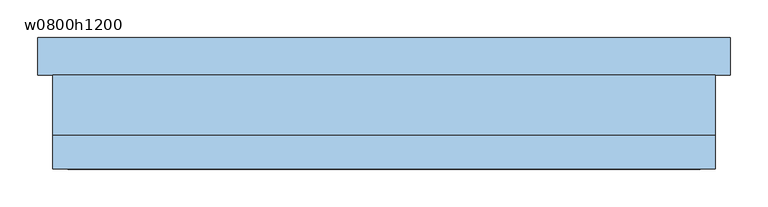
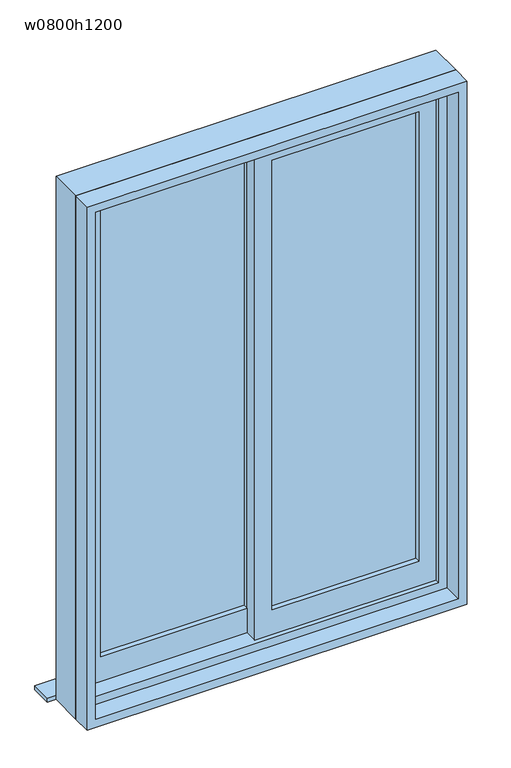
"""IFC4 building model written with IfcOpenShell, lengths in millimetres: window geometry, 引違い腰窓_2枚 : w0800h1200."""

from ifc_helpers import new_model, si_unit, frame, origin, place, context, project, spatial, polyline, outline, extrude, source, transform, mapped, element, save


def w0800h1200_be539ad6(model_context):
    return source(origin(), model_context, "Body", "SweptSolid", [
        extrude(outline(polyline([(-20.0, 12.5), (-360.0, 12.5), (-360.0, 17.5), (-20.0, 17.5), (-20.0, 12.5)])), frame((0.0, 0.0, 860.0), z_axis=(0.0, 0.0, 1.0), x_axis=(1.0, 0.0, 0.0)), (0.0, 0.0, 1.0), 1100.0),
        extrude(outline(polyline([(360.0, -17.5), (20.0, -17.5), (20.0, -12.5), (360.0, -12.5), (360.0, -17.5)])), frame((0.0, 0.0, 860.0), z_axis=(0.0, 0.0, 1.0), x_axis=(1.0, 0.0, 0.0)), (0.0, 0.0, 1.0), 1100.0),
        extrude(outline(polyline([(2000.0, -20.0), (800.0, -20.0), (800.0, 400.0), (2000.0, 400.0), (2000.0, -20.0)]), holes=[polyline([(860.0, 360.0), (860.0, 20.0), (1960.0, 20.0), (1960.0, 360.0), (860.0, 360.0)])]), frame((0.0, -30.0, 0.0), z_axis=(0.0, 1.0, 0.0), x_axis=(0.0, 0.0, 1.0)), (0.0, 0.0, 1.0), 30.0),
        extrude(outline(polyline([(2000.0, -400.0), (800.0, -400.0), (800.0, 20.0), (2000.0, 20.0), (2000.0, -400.0)]), holes=[polyline([(860.0, -20.0), (860.0, -360.0), (1960.0, -360.0), (1960.0, -20.0), (860.0, -20.0)])]), frame((0.0, 0.0, 0.0), z_axis=(0.0, 1.0, 0.0), x_axis=(0.0, 0.0, 1.0)), (0.0, 0.0, 1.0), 30.0),
        extrude(outline(polyline([(460.0, 90.0), (460.0, 40.0), (-460.0, 40.0), (-460.0, 90.0), (460.0, 90.0)])), frame((0.0, 0.0, 760.0), z_axis=(0.0, 0.0, 1.0), x_axis=(1.0, 0.0, 0.0)), (0.0, 0.0, 1.0), 10.0),
        extrude(outline(polyline([(2040.0, 440.0), (2040.0, -440.0), (760.0, -440.0), (760.0, 440.0), (2040.0, 440.0)]), holes=[polyline([(780.0, -420.0), (2020.0, -420.0), (2020.0, 420.0), (780.0, 420.0), (780.0, -420.0)])]), frame((0.0, -85.0, 0.0), z_axis=(0.0, 1.0, 0.0), x_axis=(0.0, 0.0, 1.0)), (0.0, 0.0, 1.0), 45.0),
        extrude(outline(polyline([(2040.0, -440.0), (760.0, -440.0), (760.0, 440.0), (2040.0, 440.0), (2040.0, -440.0)]), holes=[polyline([(2000.0, 400.0), (800.0, 400.0), (800.0, -400.0), (2000.0, -400.0), (2000.0, 400.0)])]), frame((0.0, -40.0, 0.0), z_axis=(0.0, 1.0, 0.0), x_axis=(0.0, 0.0, 1.0)), (0.0, 0.0, 1.0), 80.0),
    ])


if __name__ == "__main__":
    model = new_model("IFC4")
    model_context = context("Model", 3, world=origin())
    ifc_project = project(units=[si_unit("LENGTHUNIT", "METRE", prefix="MILLI")], contexts=[model_context])
    site = spatial("IfcSite", under=ifc_project)
    building = spatial("IfcBuilding", under=site)
    placement = place(None, origin())
    w0800h1200_shape = w0800h1200_be539ad6(model_context)
    element("IfcWindow", 1, ObjectType="引違い腰窓_2枚 : w0800h1200", at=placement, inside=building, context=model_context, shape_type="MappedRepresentation", body=[
        mapped(w0800h1200_shape, transform((0.0, 0.0, 0.0), x_axis=(1.0, 0.0, 0.0), y_axis=(0.0, 1.0, 0.0), z_axis=(0.0, 0.0, 1.0))),
    ])
    save(model, "model.ifc")

# Revit data of these elements
# Type "引違い腰窓_2枚 : w0800h1200"
#   Construction Type Id = "GSP4R"
#   Analytic Construction = "1/8 インチ ピルキントン一重ガラス"
#   Type Mark = "65"
#   Operation = "ダブル パネル縦"
#   Keynote = "08520.Q1"
#   Visual Light Transmittance = 0.9
#   Solar Heat Gain Coefficient = 0.86
#   Heat Transfer Coefficient (U) = 6.7069 W/(m²·K)
#   Height = 1200 mm
#   既定の腰高 = 800 mm
#   Width = 800 mm
#   額縁見附 = 20 mm
#   額縁ちり = 10 mm
#   サッシ見附 = 40 mm
#   サッシの幅 = 80 mm
#   サッシ額縁 [instance default] = none
#   サッシ本体 [instance default] = none
#   サッシガラス [instance default] = ガラス - 透明
#   Wall Closure = (empty or 0)
#   Type Comments = ""
#   Assembly Code = ""
# Element 1 (IfcWindow, "引違い腰窓_2枚 : w0800h1200")
#   Materials on its faces: "ガラス - 透明"
# Materials
#   "ガラス - 透明": class "ガラス", colour RGB 0 128 192, transparency 0.9, Cost = 0
